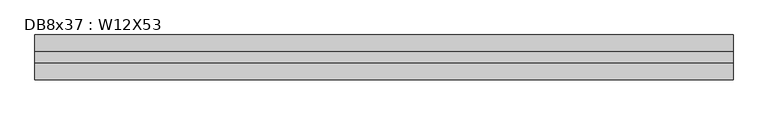
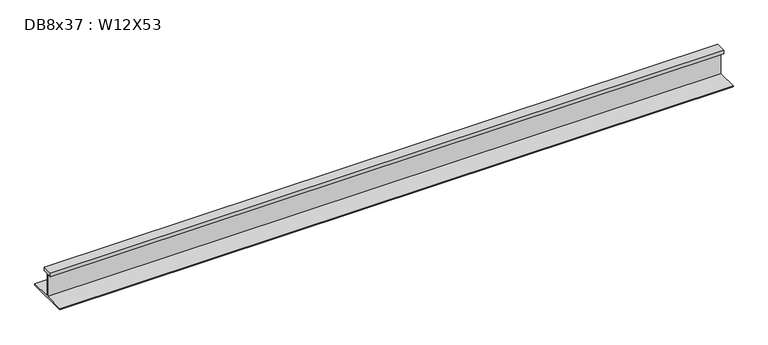
"""IFC4 building model written with IfcOpenShell, lengths in millimetres: beam geometry, DB8x37 : W12X53."""

from ifc_helpers import new_model, si_unit, frame, origin, place, context, project, spatial, polyline, outline, extrude, source, transform, mapped, element, save


def db8x37_w12x53_edb2ace5(model_context):
    return source(origin(), model_context, "Body", "SweptSolid", [
        extrude(outline(polyline([(38.1, 145.415), (38.1, 120.015), (2.921, 120.015), (2.921, -48.4505), (152.4, -48.4505), (152.4, -58.1025), (-152.4, -58.1025), (-152.4, -48.4505), (-2.921, -48.4505), (-2.921, 120.015), (-38.1, 120.015), (-38.1, 145.415), (38.1, 145.415)])), frame((-2391.029, 0.0, 0.0), z_axis=(1.0, 0.0, 0.0), x_axis=(0.0, 1.0, 0.0)), (0.0, 0.0, 1.0), 4751.959),
    ])


if __name__ == "__main__":
    model = new_model("IFC4")
    model_context = context("Model", 3, world=origin())
    ifc_project = project(units=[si_unit("LENGTHUNIT", "METRE", prefix="MILLI")], contexts=[model_context])
    site = spatial("IfcSite", under=ifc_project)
    building = spatial("IfcBuilding", under=site)
    placement = place(None, origin())
    db8x37_w12x53_shape = db8x37_w12x53_edb2ace5(model_context)
    element("IfcBeam", 1, ObjectType="DB8x37 : W12X53", at=placement, inside=building, context=model_context, shape_type="MappedRepresentation", body=[
        mapped(db8x37_w12x53_shape, transform((0.0, 0.0, 0.0), x_axis=(1.0, 0.0, 0.0), y_axis=(0.0, 1.0, 0.0), z_axis=(0.0, 0.0, 1.0))),
    ])
    save(model, "model.ifc")

# Revit data of these elements
# Type "DB8x37 : W12X53"
#   Assembly Code = "B10"
#   W = 53
#   Length [instance default] = 5' - 0"
#   bf = 0' - 10"
#   d = 1' - 0.1"
#   k = 0' - 1 3/8"
#   k2 = 0' - 0.8"
#   tf = 0' - 0.575"
#   tw = 0' - 0.345"
#   A = 0.108333 SF
#   Structural Material [instance default] = Steel ASTM A992
# Element 1 (IfcBeam, "DB8x37 : W12X53")
#   Materials on its faces: "Steel ASTM A992"
# Materials
#   "Steel ASTM A992": class "Metal", colour RGB 199 199 199, transparency 0, Description = "Structural steel 50ksi", Cost = 0
